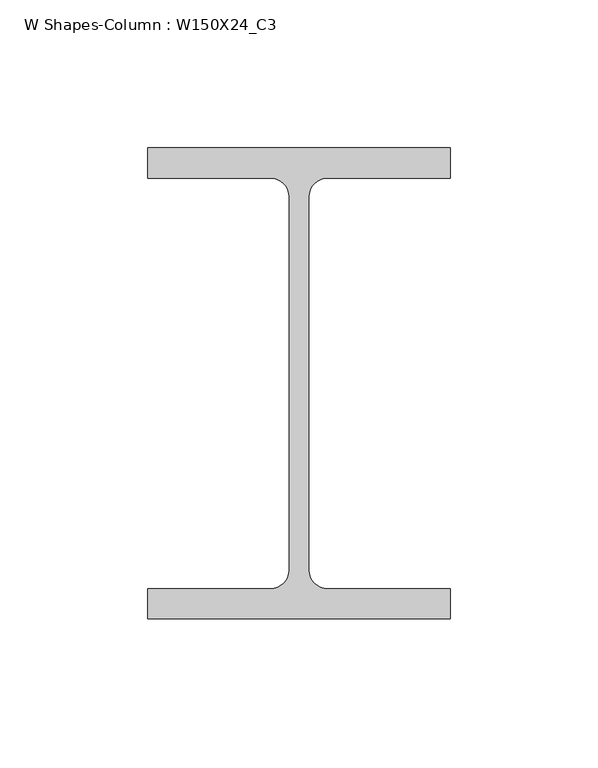
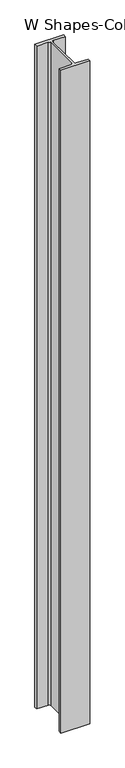
"""IFC4 building model written with IfcOpenShell, lengths in millimetres: column geometry, W Shapes-Column : W150X24_C3."""

import ifcopenshell
import ifcopenshell.guid

model = None  # the IFC model being written
_history = None  # IfcOwnerHistory: only IFC2X3 demands one
_inside = {}  # id of a spatial element -> (the spatial element, [elements in it])
_under = {}  # id of a project, library or spatial element -> (it, [spatial elements below it])
_declared = {}  # id of a project -> (the project, [libraries it declares])
_typed = {}  # id of a type object -> (the type object, [elements of that type])
_made_of = {}  # id of a material, layer set ... -> (it, [elements and type objects made of it])


def new_model(schema):
    """Start an empty IFC model of exactly this schema.

    Asked for "IFC4X3", IfcOpenShell would pick the latest addendum, in which some entities
    have other attributes; the version numbers below select the first issue.
    IFC2X3 requires an IfcOwnerHistory on every rooted entity: one is made here for all.
    """
    global model, _history
    if schema == "IFC4X3":
        model = ifcopenshell.file(schema_version=(4, 3, 0, 0))
    else:
        model = ifcopenshell.file(schema=schema)
    _inside.clear()
    _under.clear()
    _declared.clear()
    _typed.clear()
    _made_of.clear()
    _history = None
    if model.schema == "IFC2X3":
        org = make("IfcOrganization", Name="unknown")
        user = make(
            "IfcPersonAndOrganization",
            ThePerson=make("IfcPerson", FamilyName="unknown"),
            TheOrganization=org,
        )
        app = make(
            "IfcApplication",
            ApplicationDeveloper=org,
            Version="unknown",
            ApplicationFullName="unknown",
            ApplicationIdentifier="unknown",
        )
        _history = make(
            "IfcOwnerHistory",
            OwningUser=user,
            OwningApplication=app,
            ChangeAction="ADDED",
            CreationDate=0,
        )
    return model


def make(cls, **values):
    """One entity of the class cls with the attributes given. An attribute that is None is left unset."""
    return model.create_entity(
        cls, **{name: value for name, value in values.items() if value is not None}
    )


def rooted(cls, **values):
    """An entity with a GlobalId (a new one), such as an element, a storey or a relation."""
    return make(cls, GlobalId=ifcopenshell.guid.new(), OwnerHistory=_history, **values)


def si_unit(unit_type, name, prefix=None):
    """IfcSIUnit, for example si_unit("LENGTHUNIT", "METRE", prefix="MILLI")."""
    return make("IfcSIUnit", UnitType=unit_type, Prefix=prefix, Name=name)


def assignment(units):
    """IfcUnitAssignment: the units of a project."""
    return None if units is None else make("IfcUnitAssignment", Units=units)


def point(xyz):
    """IfcCartesianPoint."""
    return None if xyz is None else make("IfcCartesianPoint", Coordinates=xyz)


def direction(xyz):
    """IfcDirection."""
    return None if xyz is None else make("IfcDirection", DirectionRatios=xyz)


def frame(location, z_axis=None, x_axis=None):
    """IfcAxis2Placement3D, a coordinate frame: its origin and axes. An axis left out is left unset."""
    return make(
        "IfcAxis2Placement3D",
        Location=point(location),
        Axis=direction(z_axis),
        RefDirection=direction(x_axis),
    )


def frame_2d(location, x_axis=None):
    """IfcAxis2Placement2D, a coordinate frame in the plane: its origin and x axis."""
    return make(
        "IfcAxis2Placement2D", Location=point(location), RefDirection=direction(x_axis)
    )


def origin():
    """The frame at (0, 0, 0) with its axes left unset."""
    return frame((0.0, 0.0, 0.0))


def place(relative_to, where):
    """IfcLocalPlacement: puts the frame where relative to a parent placement (None: the world)."""
    return make(
        "IfcLocalPlacement", PlacementRelTo=relative_to, RelativePlacement=where
    )


def context(
    kind, dimensions, precision=None, world=None, true_north=None, identifier=None
):
    """IfcGeometricRepresentationContext, for example the 3D "Model" context."""
    return make(
        "IfcGeometricRepresentationContext",
        ContextIdentifier=identifier,
        ContextType=kind,
        CoordinateSpaceDimension=dimensions,
        Precision=precision,
        WorldCoordinateSystem=world,
        TrueNorth=true_north,
    )


def project(units=None, contexts=None):
    """IfcProject with its units and contexts."""
    return rooted(
        "IfcProject",
        Name="project",
        RepresentationContexts=contexts,
        UnitsInContext=assignment(units),
    )


def spatial(cls, under=None, at=None, **own):
    """A site, building, storey or space (cls), placed at a placement, below another one or the project."""
    s = rooted(cls, ObjectPlacement=at, **own)
    if under is not None:
        _under.setdefault(under.id(), (under, []))[1].append(s)
    return s


def polyline(points):
    """IfcPolyline through the points."""
    return make("IfcPolyline", Points=[point(p) for p in points])


def circle_curve(where, radius):
    """IfcCircle in the frame where."""
    return make("IfcCircle", Position=where, Radius=radius)


def trimmed(basis, trim1, trim2, sense, master):
    """IfcTrimmedCurve: the piece of a basis curve between two trims."""
    return make(
        "IfcTrimmedCurve",
        BasisCurve=basis,
        Trim1=trim1,
        Trim2=trim2,
        SenseAgreement=sense,
        MasterRepresentation=master,
    )


def segment(curve, same_sense, transition):
    """IfcCompositeCurveSegment."""
    return make(
        "IfcCompositeCurveSegment",
        Transition=transition,
        SameSense=same_sense,
        ParentCurve=curve,
    )


def composite_curve(segments, self_intersect=None):
    """IfcCompositeCurve: segments joined end to end."""
    return make("IfcCompositeCurve", Segments=segments, SelfIntersect=self_intersect)


def outline(outer, holes=None, kind="AREA"):
    """IfcArbitraryClosedProfileDef: a profile drawn as a closed curve; with holes, ...WithVoids."""
    if holes is None:
        return make("IfcArbitraryClosedProfileDef", ProfileType=kind, OuterCurve=outer)
    return make(
        "IfcArbitraryProfileDefWithVoids",
        ProfileType=kind,
        OuterCurve=outer,
        InnerCurves=holes,
    )


def extrude(swept, where, along, depth):
    """IfcExtrudedAreaSolid: the profile swept, set in the frame where, extruded along a direction by depth."""
    return make(
        "IfcExtrudedAreaSolid",
        SweptArea=swept,
        Position=where,
        ExtrudedDirection=direction(along),
        Depth=depth,
    )


def shape(context_of_items, identifier, shape_type, items):
    """IfcShapeRepresentation: the items that make up one representation, for example the "Body"."""
    return make(
        "IfcShapeRepresentation",
        ContextOfItems=context_of_items,
        RepresentationIdentifier=identifier,
        RepresentationType=shape_type,
        Items=items,
    )


def source(mapping_origin, context_of_items, identifier, shape_type, items):
    """IfcRepresentationMap: a shape defined once, which mapped items show again and again."""
    return make(
        "IfcRepresentationMap",
        MappingOrigin=mapping_origin,
        MappedRepresentation=shape(context_of_items, identifier, shape_type, items),
    )


def transform(
    local_origin,
    x_axis=None,
    y_axis=None,
    z_axis=None,
    scale=None,
    scale2=None,
    scale3=None,
    uniform=True,
):
    """IfcCartesianTransformationOperator3D, or its non-uniform kind. x_axis, y_axis, z_axis: its Axis1, 2, 3."""
    if uniform:
        return make(
            "IfcCartesianTransformationOperator3D",
            Axis1=direction(x_axis),
            Axis2=direction(y_axis),
            LocalOrigin=point(local_origin),
            Scale=scale,
            Axis3=direction(z_axis),
        )
    return make(
        "IfcCartesianTransformationOperator3DnonUniform",
        Axis1=direction(x_axis),
        Axis2=direction(y_axis),
        LocalOrigin=point(local_origin),
        Scale=scale,
        Axis3=direction(z_axis),
        Scale2=scale2,
        Scale3=scale3,
    )


def mapped(mapping_source, mapping_target):
    """IfcMappedItem: shows the shape of a source again, moved by a transform."""
    return make(
        "IfcMappedItem", MappingSource=mapping_source, MappingTarget=mapping_target
    )


def made_of(thing, what):
    """Note that an element or type object is made of a material, layer set ...; save() writes the relation."""
    if what is not None:
        _made_of.setdefault(what.id(), (what, []))[1].append(thing)
    return thing


def element(
    cls,
    number,
    at=None,
    inside=None,
    cuts=None,
    type_object=None,
    material=None,
    context=None,
    identifier="Body",
    shape_type=None,
    held_by="IfcProductDefinitionShape",
    body=None,
    shapes=None,
    **own,
):
    """One element of the class cls, such as IfcWall. Its Tag is "e" and its number.

    at: its placement. inside: the storey or other place that contains it. cuts: it is an
    opening in that element (IfcRelVoidsElement). A single representation is given by context,
    identifier, shape_type and body (its items); several are given by shapes. held_by: the class
    of the entity that holds the representations. save() writes the other relations.
    """
    e = rooted(cls, Tag="e%d" % number, ObjectPlacement=at, **own)
    if body is not None:
        shapes = [shape(context, identifier, shape_type, body)]
    if shapes is not None:
        e.Representation = make(held_by, Representations=shapes)
    if inside is not None:
        _inside.setdefault(inside.id(), (inside, []))[1].append(e)
    if cuts is not None:
        rooted(
            "IfcRelVoidsElement", RelatingBuildingElement=cuts, RelatedOpeningElement=e
        )
    if type_object is not None:
        _typed.setdefault(type_object.id(), (type_object, []))[1].append(e)
    return made_of(e, material)


def aggregate(whole, parts):
    """IfcRelAggregates: a whole, such as a stair, and the parts it consists of."""
    return rooted("IfcRelAggregates", RelatingObject=whole, RelatedObjects=parts)


def save(model, path):
    """Write the relations noted so far, then the file.

    IfcRelAggregates (storeys below a building ...), IfcRelContainedInSpatialStructure (elements
    in a storey), IfcRelDefinesByType, IfcRelAssociatesMaterial and IfcRelDeclares: one each for
    every whole, place, type object, material and project.
    """
    for whole, parts in _under.values():
        aggregate(whole, parts)
    for where, things in _inside.values():
        rooted(
            "IfcRelContainedInSpatialStructure",
            RelatedElements=things,
            RelatingStructure=where,
        )
    for kind, things in _typed.values():
        rooted("IfcRelDefinesByType", RelatedObjects=things, RelatingType=kind)
    for what, things in _made_of.values():
        rooted("IfcRelAssociatesMaterial", RelatedObjects=things, RelatingMaterial=what)
    for by, libraries in _declared.values():
        rooted("IfcRelDeclares", RelatingContext=by, RelatedDefinitions=libraries)
    model.write(path)


def w_shapes_column_w150x24_c3_35ee5e78(model_context):
    return source(origin(), model_context, "Body", "SweptSolid", [
        extrude(outline(composite_curve([segment(polyline([(51.181, 79.756), (51.181, 69.469), (9.652, 69.469)]), True, "CONTINUOUS"), segment(trimmed(circle_curve(frame_2d((9.652, 63.119)), 6.35), [point((9.652, 69.469))], [point((3.302, 63.119))], True, "CARTESIAN"), True, "CONTINUOUS"), segment(polyline([(3.302, 63.119), (3.302, -63.119)]), True, "CONTINUOUS"), segment(trimmed(circle_curve(frame_2d((9.652, -63.119)), 6.35), [point((3.302, -63.119))], [point((9.652, -69.469))], True, "CARTESIAN"), True, "CONTINUOUS"), segment(polyline([(9.652, -69.469), (51.181, -69.469), (51.181, -79.756), (-51.181, -79.756), (-51.181, -69.469), (-9.652, -69.469)]), True, "CONTINUOUS"), segment(trimmed(circle_curve(frame_2d((-9.652, -63.119)), 6.35), [point((-9.652, -69.469))], [point((-3.302, -63.119))], True, "CARTESIAN"), True, "CONTINUOUS"), segment(polyline([(-3.302, -63.119), (-3.302, 63.119)]), True, "CONTINUOUS"), segment(trimmed(circle_curve(frame_2d((-9.652, 63.119)), 6.35), [point((-3.302, 63.119))], [point((-9.652, 69.469))], True, "CARTESIAN"), True, "CONTINUOUS"), segment(polyline([(-9.652, 69.469), (-51.181, 69.469), (-51.181, 79.756), (51.181, 79.756)]), True, "CONTINUOUS")], self_intersect=False)), frame((0.0, 0.0, 10066.0), z_axis=(0.0, 0.0, 1.0), x_axis=(1.0, 0.0, 0.0)), (0.0, 0.0, 1.0), 2484.0),
    ])


if __name__ == "__main__":
    model = new_model("IFC4")
    model_context = context("Model", 3, world=origin())
    ifc_project = project(units=[si_unit("LENGTHUNIT", "METRE", prefix="MILLI")], contexts=[model_context])
    site = spatial("IfcSite", under=ifc_project)
    building = spatial("IfcBuilding", under=site)
    placement = place(None, origin())
    w_shapes_column_w150x24_c3_shape = w_shapes_column_w150x24_c3_35ee5e78(model_context)
    element("IfcColumn", 1, ObjectType="W Shapes-Column : W150X24_C3", at=placement, inside=building, context=model_context, shape_type="MappedRepresentation", body=[
        mapped(w_shapes_column_w150x24_c3_shape, transform((0.0, 0.0, 0.0), x_axis=(1.0, 0.0, 0.0), y_axis=(0.0, 1.0, 0.0), z_axis=(0.0, 0.0, 1.0))),
    ])
    save(model, "model.ifc")

# Revit data of these elements
# Type "W Shapes-Column : W150X24_C3"
#   Section Name Key = "W6x16"
#   Assembly Code = "B10"
#   Width = 10.2362 cm
#   Web Thickness = 0.6604 cm
#   Web Fillet = 0.635 cm
#   Warping Constant = 10258.1 cm⁶
#   Torsional Moment of Inertia = 9.28196 cm⁴
#   Section Area = 30.5806 cm²
#   Plastic Modulus weak axis = 55.5521 cm³
#   Plastic Modulus strong axis = 191.729 cm³
#   Perimeter = 0.704088 m²/m
#   Nominal Weight = 23.8106 kgf/m
#   Moment of Inertia weak axis = 184.391 cm⁴
#   Moment of Inertia strong axis = 1336.10 cm⁴
#   Height = 15.9512 cm
#   Flange Thickness = 1.0287 cm
#   Elastic Modulus weak axis = 36.0515 cm³
#   Elastic Modulus strong axis = 167.148 cm³
#   Clear Web Height = 19.05 cm
#   Centroid Vertical = 7.9756 cm
#   Centroid Horizontal = 5.1181 cm
#   Bolt Spacing = 5.715 cm
#   Structural Material [instance default] = Steel ASTM A992
#   Principal Axes Angle = 0
# Element 1 (IfcColumn, "W Shapes-Column : W150X24_C3")
#   Structural Material = none
# Materials
#   "Steel ASTM A992": class "Metal", colour RGB 199 199 199, transparency 0, Description = "Structural steel 50ksi", Cost = 0
